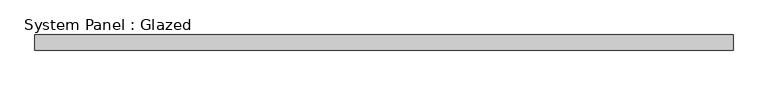
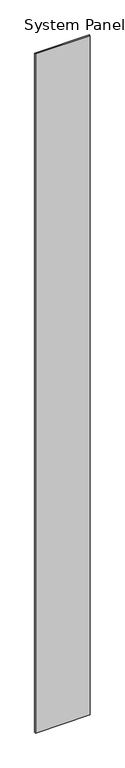
"""IFC4 building model written with IfcOpenShell, lengths in millimetres: plate geometry, System Panel : Glazed."""

from ifc_helpers import new_model, si_unit, origin, origin_with_axes, place, context, project, spatial, polyline, outline, extrude, source, transform, mapped, element, save


def system_panel_glazed_1400d148(model_context):
    return source(origin(), model_context, "Body", "SweptSolid", [
        extrude(outline(polyline([(569.3200969, 19.05), (-569.3200969, 19.05), (-569.3200969, 44.45), (569.3200969, 44.45), (569.3200969, 19.05)])), origin_with_axes(), (0.0, 0.0, 1.0), 14960.6),
    ])


if __name__ == "__main__":
    model = new_model("IFC4")
    model_context = context("Model", 3, world=origin())
    ifc_project = project(units=[si_unit("LENGTHUNIT", "METRE", prefix="MILLI")], contexts=[model_context])
    site = spatial("IfcSite", under=ifc_project)
    building = spatial("IfcBuilding", under=site)
    placement = place(None, origin())
    system_panel_glazed_shape = system_panel_glazed_1400d148(model_context)
    element("IfcPlate", 1, ObjectType="System Panel : Glazed", at=placement, inside=building, context=model_context, shape_type="MappedRepresentation", body=[
        mapped(system_panel_glazed_shape, transform((0.0, 0.0, 0.0), x_axis=(1.0, 0.0, 0.0), y_axis=(0.0, 1.0, 0.0), z_axis=(0.0, 0.0, 1.0))),
    ])
    save(model, "model.ifc")

# Revit data of these elements
# Type "System Panel : Glazed"
#   Construction Type Id = "GSP4R"
#   Analytic Construction = "1/8 in Pilkington single glazing"
#   Visual Light Transmittance = 0.9
#   Solar Heat Gain Coefficient = 0.86
#   Heat Transfer Coefficient (U) = 1.18115 BTU/(h·ft²·°F)
#   Define Thermal Properties by = 1
# Element 1 (IfcPlate, "System Panel : Glazed")
#   Materials on its faces: "Glass"
# Materials
#   "Glass": class "Glass", colour RGB 0 128 192, transparency 0.75, Description = "Soda Lime Glass", Cost = 0
